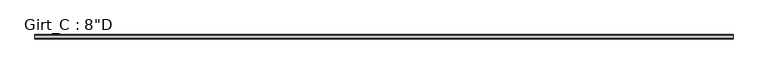
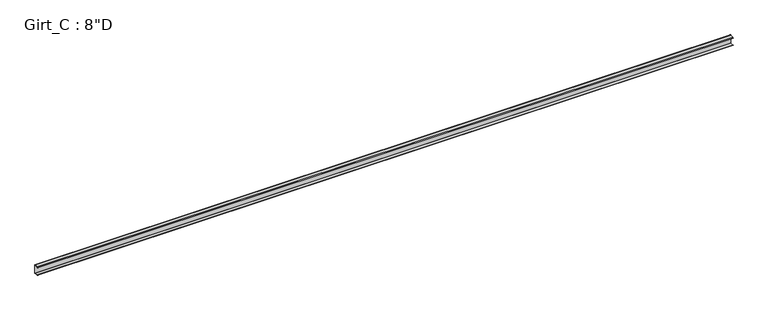
"""IFC4 building model written with IfcOpenShell, lengths in millimetres: beam geometry."""

from ifc_helpers import new_model, si_unit, point, frame, frame_2d, origin, place, context, project, spatial, polyline, circle_curve, trimmed, segment, composite_curve, outline, extrude, source, transform, mapped, element, save


def beam_22635dde(model_context):
    return source(origin(), model_context, "Body", "SweptSolid", [
        extrude(outline(composite_curve([segment(polyline([(-87.5109375, 101.6), (-3.3734375, 101.6)]), True, "CONTINUOUS"), segment(trimmed(circle_curve(frame_2d((-3.3734375, 96.8375)), 4.7625), [point((-3.3734375, 101.6))], [point((1.3890625, 96.8375))], False, "CARTESIAN"), True, "CONTINUOUS"), segment(polyline([(1.3890625, 96.8375), (1.3890625, -96.8375)]), True, "CONTINUOUS"), segment(trimmed(circle_curve(frame_2d((-3.3734375, -96.8375)), 4.7625), [point((1.3890625, -96.8375))], [point((-3.3734375, -101.6))], False, "CARTESIAN"), True, "CONTINUOUS"), segment(polyline([(-3.3734375, -101.6), (-87.5109375, -101.6), (-99.7792647, -86.979177), (-97.6510975, -85.1934327), (-86.2154765, -98.821875), (-3.2694106, -98.821875)]), True, "CONTINUOUS"), segment(trimmed(circle_curve(frame_2d((-3.3748024, -96.8389339)), 1.9857399), [point((-3.2694106, -98.821875))], [point((-1.3890625, -96.8389339))], True, "CARTESIAN"), True, "CONTINUOUS"), segment(polyline([(-1.3890625, -96.8389339), (-1.3890625, 96.8381931)]), True, "CONTINUOUS"), segment(trimmed(circle_curve(frame_2d((-3.3741066, 96.8381931)), 1.9850441), [point((-1.3890625, 96.8381931))], [point((-3.3005807, 98.821875))], True, "CARTESIAN"), True, "CONTINUOUS"), segment(polyline([(-3.3005807, 98.821875), (-86.2154765, 98.821875), (-97.6278742, 85.221109), (-99.7560415, 87.0068534), (-87.5109375, 101.6)]), True, "CONTINUOUS")], self_intersect=False)), frame((-7996.2976659, 0.0, 0.0), z_axis=(1.0, 0.0, 0.0), x_axis=(0.0, 1.0, 0.0)), (0.0, 0.0, 1.0), 15992.5953317),
    ])


if __name__ == "__main__":
    model = new_model("IFC4")
    model_context = context("Model", 3, world=origin())
    ifc_project = project(units=[si_unit("LENGTHUNIT", "METRE", prefix="MILLI")], contexts=[model_context])
    site = spatial("IfcSite", under=ifc_project)
    building = spatial("IfcBuilding", under=site)
    placement = place(None, origin())
    beam_shape = beam_22635dde(model_context)
    element("IfcBeam", 1, ObjectType="Girt_C : 8\"D", at=placement, inside=building, context=model_context, shape_type="MappedRepresentation", body=[
        mapped(beam_shape, transform((0.0, 0.0, 0.0), x_axis=(1.0, 0.0, 0.0), y_axis=(0.0, 1.0, 0.0), z_axis=(0.0, 0.0, 1.0))),
    ])
    save(model, "model.ifc")

# Revit data of these elements
# Type "Girt_C : 8\"D"
#   half leg = 0' - 1 3/4"
#   Web_Thickness = 0' - 0 7/64"
#   Length [instance default] = 10' - 0"
#   Leg_1 = 0' - 3 1/2"
#   Height = 0' - 8"
#   Structural Material [instance default] = none
# Element 1 (IfcBeam, "Girt_C : 8\"D")
#   Structural Material = GALVANIZED 'CEE' SECTION (8.0x3.5C - SEE STRUCT. DWGS)
#   Materials on its faces: "GALVANIZED 'CEE' SECTION (8.0x3.5C - SEE STRUCT. DWGS)"
# Materials
#   "GALVANIZED 'CEE' SECTION (8.0x3.5C - SEE STRUCT. DWGS)": class "Metal", colour RGB 137 146 153, transparency 0, Description = "Steel, mill finish", Cost = 0
